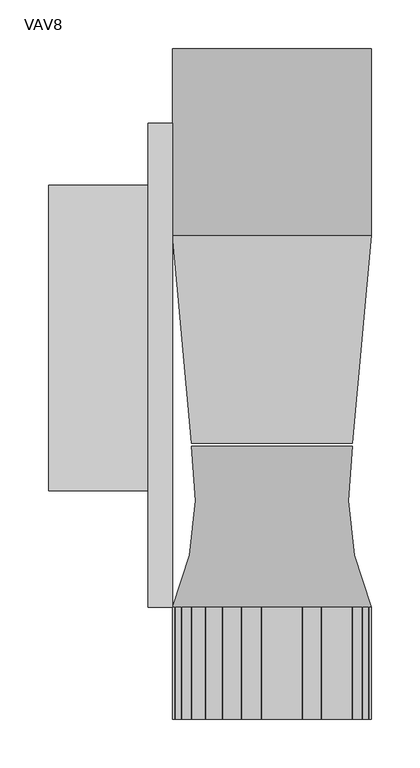
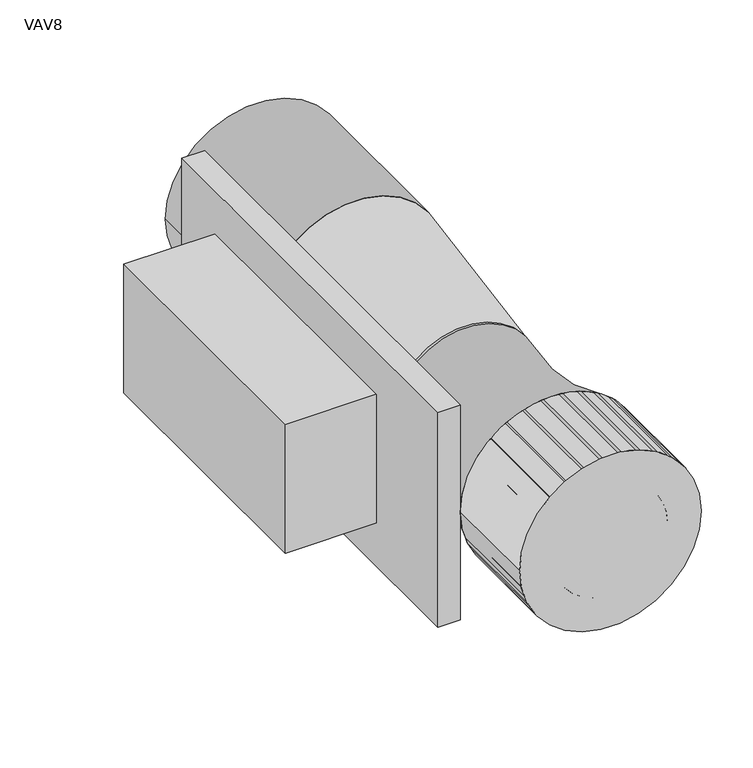
"""IFC4 building model written with IfcOpenShell, lengths in millimetres: proxy geometry, VAV8 : PValve200."""

from ifc_helpers import new_model, si_unit, point, frame, origin, origin_2d, place, context, project, spatial, polyline, circle_curve, ellipse_curve, trimmed, segment, composite_curve, outline, extrude, source, transform, mapped, element, save
from ifc_brep_helpers import plane_surface, revolved_surface, advanced_brep


def vav8_1438daf9(model_context):
    return source(origin(), model_context, "Body", "SolidModel", [
        extrude(outline(composite_curve([segment(trimmed(circle_curve(origin_2d(), 101.6), [point((0.0, 101.6))], [point((0.0, -101.6))], False, "CARTESIAN"), True, "CONTINUOUS"), segment(trimmed(circle_curve(origin_2d(), 101.6), [point((0.0, -101.6))], [point((0.0, 101.6))], False, "CARTESIAN"), True, "CONTINUOUS")], self_intersect=False)), frame((0.0, 0.0, 0.0), z_axis=(0.0, 1.0, 0.0), x_axis=(0.0, 0.0, 1.0)), (0.0, 0.0, 1.0), 114.3),
        advanced_brep(
        [(101.6, 114.3, 0.0), (63.5, 114.3, 0.0), (-63.5, 114.3, 0.0), (-101.6, 114.3, 0.0), (-82.55, 279.4, 0.0), (-63.5, 279.4, 0.0), (63.5, 279.4, 0.0), (82.55, 279.4, 0.0)],
        [
            (0, 1),
            (1, 2, circle_curve(frame((0.0, 114.3, 0.0), z_axis=(0.0, 1.0, 0.0), x_axis=(1.0, 0.0, 0.0)), 63.5)),
            (2, 3),
            (3, 0, circle_curve(frame((0.0, 114.3, 0.0), z_axis=(0.0, -1.0, 0.0), x_axis=(1.0, 0.0, 0.0)), 101.6)),
            (2, 1, circle_curve(frame((0.0, 114.3, 0.0), z_axis=(0.0, 1.0, 0.0), x_axis=(1.0, 0.0, 0.0)), 63.5)),
            (0, 3, circle_curve(frame((0.0, 114.3, 0.0), z_axis=(0.0, -1.0, 0.0), x_axis=(1.0, 0.0, 0.0)), 101.6)),
            (4, 5),
            (5, 6, circle_curve(frame((0.0, 279.4, 0.0), z_axis=(0.0, -1.0, 0.0), x_axis=(1.0, 0.0, 0.0)), 63.5)),
            (6, 7),
            (7, 4, circle_curve(frame((0.0, 279.4, 0.0), z_axis=(0.0, 1.0, 0.0), x_axis=(1.0, 0.0, 0.0)), 82.55)),
            (6, 5, circle_curve(frame((0.0, 279.4, 0.0), z_axis=(0.0, -1.0, 0.0), x_axis=(1.0, 0.0, 0.0)), 63.5)),
            (4, 7, circle_curve(frame((0.0, 279.4, 0.0), z_axis=(0.0, 1.0, 0.0), x_axis=(1.0, 0.0, 0.0)), 82.55)),
            (5, 2),
            (1, 6),
            (3, 4, circle_curve(frame((-368.6011377, 228.756862, 0.0), z_axis=(0.0, 0.0, 1.0), x_axis=(-1.0, 0.0, 0.0)), 290.4995367)),
            (7, 0, circle_curve(frame((368.6011377, 228.756862, 0.0), z_axis=(0.0, 0.0, 1.0), x_axis=(1.0, 0.0, 0.0)), 290.4995367)),
        ],
        [
            plane_surface(frame((0.0, 114.3, 0.0), z_axis=(0.0, -1.0, 0.0), x_axis=(1.0, 0.0, 0.0))),
            plane_surface(frame((0.0, 279.4, 0.0), z_axis=(0.0, 1.0, 0.0), x_axis=(1.0, 0.0, 0.0))),
            revolved_surface(polyline([(63.5, 279.4, 0.0), (63.5, 114.3, 0.0)]), (0.0, 0.0, 0.0), (0.0, 1.0, 0.0)),
            revolved_surface(trimmed(ellipse_curve(frame((368.6011377, 228.756862, 0.0), z_axis=(0.0, 0.0, 1.0), x_axis=(1.0, 0.0, 0.0)), 290.4995367, 290.4995367), [point((82.55, 279.4, 0.0))], [point((101.6, 114.3, 0.0))], True, "CARTESIAN"), (0.0, 114.3, 0.0), (0.0, -1.0, 0.0)),
        ],
        [
            (0, [[1, 2, 3, 4]]),
            (0, [[-3, 5, -1, 6]]),
            (1, [[7, 8, 9, 10]]),
            (1, [[-9, 11, -7, 12]]),
            (2, [[-8, 13, -2, 14]]),
            (2, [[-5, -13, -11, -14]]),
            (3, [[15, -10, 16, -4]]),
            (3, [[-16, -12, -15, -6]]),
        ],
    ),
        extrude(outline(composite_curve([segment(trimmed(circle_curve(origin_2d(), 101.6), [point((0.0, -101.6))], [point((0.0, 101.6))], False, "CARTESIAN"), True, "CONTINUOUS"), segment(trimmed(circle_curve(origin_2d(), 101.6), [point((0.0, 101.6))], [point((0.0, -101.6))], False, "CARTESIAN"), True, "CONTINUOUS")], self_intersect=False), holes=[composite_curve([segment(trimmed(circle_curve(origin_2d(), 63.5), [point((0.0, -63.5))], [point((0.0, 63.5))], True, "CARTESIAN"), True, "CONTINUOUS"), segment(trimmed(circle_curve(origin_2d(), 63.5), [point((0.0, 63.5))], [point((0.0, -63.5))], True, "CARTESIAN"), True, "CONTINUOUS")], self_intersect=False)]), frame((0.0, 0.0, 0.0), z_axis=(0.0, 1.0, 0.0), x_axis=(0.0, 0.0, 1.0)), (0.0, 0.0, 1.0), 114.3),
        extrude(outline(polyline([(-228.6, 546.1), (-127.0, 546.1), (-127.0, 233.5601781), (-228.6, 233.5601781), (-228.6, 546.1)])), frame((0.0, 0.0, -76.2), z_axis=(0.0, 0.0, 1.0), x_axis=(1.0, 0.0, 0.0)), (0.0, 0.0, 1.0), 152.4),
        extrude(outline(polyline([(-101.6, 609.6), (-101.6, 114.3), (-127.0, 114.3), (-127.0, 609.6), (-101.6, 609.6)])), frame((0.0, 0.0, -127.0), z_axis=(0.0, 0.0, 1.0), x_axis=(1.0, 0.0, 0.0)), (0.0, 0.0, 1.0), 254.0),
        extrude(outline(composite_curve([segment(trimmed(circle_curve(origin_2d(), 101.6), [point((0.0, -101.6))], [point((0.0, 101.6))], False, "CARTESIAN"), True, "CONTINUOUS"), segment(trimmed(circle_curve(origin_2d(), 101.6), [point((0.0, 101.6))], [point((0.0, -101.6))], False, "CARTESIAN"), True, "CONTINUOUS")], self_intersect=False)), frame((0.0, 495.3, 0.0), z_axis=(0.0, 1.0, 0.0), x_axis=(0.0, 0.0, 1.0)), (0.0, 0.0, 1.0), 190.5),
        advanced_brep(
        [(0.0, 495.3, 0.0), (101.6, 495.3, 0.0), (-101.6, 495.3, 0.0), (82.55, 282.3810845, 0.0), (0.0, 282.3810845, 0.0), (-82.55, 282.3810845, 0.0)],
        [
            (0, 1),
            (1, 2, circle_curve(frame((0.0, 495.3, 0.0), z_axis=(0.0, 1.0, 0.0), x_axis=(-1.0, 0.0, 0.0)), 101.6)),
            (2, 0),
            (2, 1, circle_curve(frame((0.0, 495.3, 0.0), z_axis=(0.0, 1.0, 0.0), x_axis=(-1.0, 0.0, 0.0)), 101.6)),
            (3, 4),
            (4, 5),
            (5, 3, circle_curve(frame((0.0, 282.3810845, 0.0), z_axis=(0.0, -1.0, 0.0), x_axis=(-1.0, 0.0, 0.0)), 82.55)),
            (3, 5, circle_curve(frame((0.0, 282.3810845, 0.0), z_axis=(0.0, -1.0, 0.0), x_axis=(-1.0, 0.0, 0.0)), 82.55)),
            (1, 3),
            (5, 2),
        ],
        [
            plane_surface(frame((0.0, 495.3, 0.0), z_axis=(0.0, 1.0, 0.0), x_axis=(-1.0, 0.0, 0.0))),
            plane_surface(frame((0.0, 282.3810845, 0.0), z_axis=(0.0, -1.0, 0.0), x_axis=(-1.0, 0.0, 0.0))),
            revolved_surface(polyline([(-82.55, 282.3810845, 0.0), (-101.6, 495.3, 0.0)]), (0.0, 279.4, 0.0), (0.0, 1.0, 0.0)),
        ],
        [
            (0, [[1, 2, 3]]),
            (0, [[-3, 4, -1]]),
            (1, [[5, 6, 7]]),
            (1, [[-6, -5, 8]]),
            (2, [[9, -7, 10, -2]]),
            (2, [[-10, -8, -9, -4]]),
        ],
    ),
    ])


if __name__ == "__main__":
    model = new_model("IFC4")
    model_context = context("Model", 3, world=origin())
    ifc_project = project(units=[si_unit("LENGTHUNIT", "METRE", prefix="MILLI")], contexts=[model_context])
    site = spatial("IfcSite", under=ifc_project)
    building = spatial("IfcBuilding", under=site)
    placement = place(None, origin())
    vav8_shape = vav8_1438daf9(model_context)
    element("IfcBuildingElementProxy", 1, Name="VAV8 : PValve200", ObjectType="VAV8 : PValve200", at=placement, inside=building, context=model_context, shape_type="MappedRepresentation", body=[
        mapped(vav8_shape, transform((0.0, 0.0, 0.0), x_axis=(1.0, 0.0, 0.0), y_axis=(0.0, 1.0, 0.0), z_axis=(0.0, 0.0, 1.0))),
    ])
    save(model, "model.ifc")

# Revit data of these elements
# Type "VAV8 : PValve200"
#   DuctSAUP = 0"
#   DuctSADN = 0"
#   Assembly Code = ""
